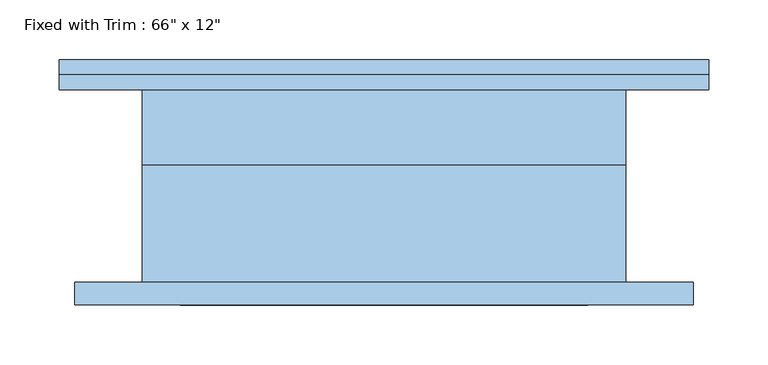
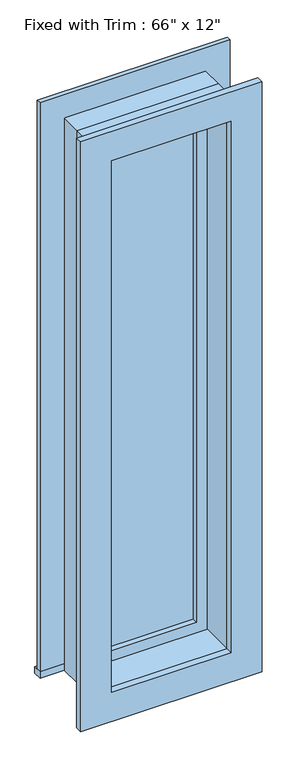
"""IFC4 building model written with IfcOpenShell, lengths in millimetres: window geometry."""

from ifc_helpers import new_model, si_unit, frame, origin, place, context, project, spatial, polyline, outline, extrude, source, transform, mapped, element, save


def window_78a8b392(model_context):
    return source(origin(), model_context, "Body", "SweptSolid", [
        extrude(outline(polyline([(-311.15, 106.3625), (234.95, 106.3625), (234.95, 80.9625), (-311.15, 80.9625), (-311.15, 106.3625)])), frame((0.0, 0.0, 304.8), z_axis=(0.0, 0.0, 1.0), x_axis=(1.0, 0.0, 0.0)), (0.0, 0.0, 1.0), 19.05),
        extrude(outline(polyline([(1962.15, -222.25), (1962.15, 146.05), (323.85, 146.05), (323.85, 234.95), (2051.05, 234.95), (2051.05, -311.15), (323.85, -311.15), (323.85, -222.25), (1962.15, -222.25)])), frame((0.0, 80.9625, 0.0), z_axis=(0.0, 1.0, 0.0), x_axis=(0.0, 0.0, 1.0)), (0.0, 0.0, 1.0), 12.7),
        extrude(outline(polyline([(2038.35, 222.25), (2038.35, -298.45), (247.65, -298.45), (247.65, 222.25), (2038.35, 222.25)]), holes=[polyline([(1949.45, 133.35), (336.55, 133.35), (336.55, -209.55), (1949.45, -209.55), (1949.45, 133.35)])]), frame((0.0, -100.0125, 0.0), z_axis=(0.0, 1.0, 0.0), x_axis=(0.0, 0.0, 1.0)), (0.0, 0.0, 1.0), 19.05),
        extrude(outline(polyline([(101.6, 33.3375), (-177.8, 33.3375), (-177.8, 46.0375), (101.6, 46.0375), (101.6, 33.3375)])), frame((0.0, 0.0, 368.3), z_axis=(0.0, 0.0, 1.0), x_axis=(1.0, 0.0, 0.0)), (0.0, 0.0, 1.0), 1549.4),
        extrude(outline(polyline([(1962.15, -222.25), (323.85, -222.25), (323.85, 146.05), (1962.15, 146.05), (1962.15, -222.25)]), holes=[polyline([(1917.7, -177.8), (1917.7, 101.6), (368.3, 101.6), (368.3, -177.8), (1917.7, -177.8)])]), frame((0.0, 17.4625, 0.0), z_axis=(0.0, 1.0, 0.0), x_axis=(0.0, 0.0, 1.0)), (0.0, 0.0, 1.0), 44.45),
        extrude(outline(polyline([(1981.2, -241.3), (304.8, -241.3), (304.8, 165.1), (1981.2, 165.1), (1981.2, -241.3)]), holes=[polyline([(1949.45, -209.55), (1949.45, 133.35), (336.55, 133.35), (336.55, -209.55), (1949.45, -209.55)])]), frame((0.0, -80.9625, 0.0), z_axis=(0.0, 1.0, 0.0), x_axis=(0.0, 0.0, 1.0)), (0.0, 0.0, 1.0), 98.425),
        extrude(outline(polyline([(1981.2, 165.1), (1981.2, -241.3), (304.8, -241.3), (304.8, 165.1), (1981.2, 165.1)]), holes=[polyline([(1962.15, 146.05), (323.85, 146.05), (323.85, -222.25), (1962.15, -222.25), (1962.15, 146.05)])]), frame((0.0, 17.4625, 0.0), z_axis=(0.0, 1.0, 0.0), x_axis=(0.0, 0.0, 1.0)), (0.0, 0.0, 1.0), 63.5),
    ])


if __name__ == "__main__":
    model = new_model("IFC4")
    model_context = context("Model", 3, world=origin())
    ifc_project = project(units=[si_unit("LENGTHUNIT", "METRE", prefix="MILLI")], contexts=[model_context])
    site = spatial("IfcSite", under=ifc_project)
    building = spatial("IfcBuilding", under=site)
    placement = place(None, origin())
    window_shape = window_78a8b392(model_context)
    element("IfcWindow", 1, ObjectType="Fixed with Trim : 66\" x 12\"", at=placement, inside=building, context=model_context, shape_type="MappedRepresentation", body=[
        mapped(window_shape, transform((0.0, 0.0, 0.0), x_axis=(1.0, 0.0, 0.0), y_axis=(0.0, 1.0, 0.0), z_axis=(0.0, 0.0, 1.0))),
    ])
    save(model, "model.ifc")

# Revit data of these elements
# Type "Fixed with Trim : 66\" x 12\""
#   Type Mark = "54"
#   COBie.Type.CreatedBy = "doug.wood@us.ibm.com"
#   COBie.Type.CreatedOn = "2016-04-14T02:07:26"
#   COBie.Type.Name = "Windows_Fixed with Trim_66\" x 12\"_54"
#   COBie.Type.Category = "23-30 20 17 11 : Fixed Windows"
#   COBie.Type.Description = "Fixed with Trim_66\" x 12\""
#   COBie.Type.Manufacturer = ""
#   COBie.Type.ModelNumber = ""
#   Construction Type Id = "GSP4R"
#   Assembly Code = "B2020100"
#   Analytic Construction = "1/8 in Pilkington single glazing"
#   COBie.Type.ReplacementCost = 0
#   Visual Light Transmittance = 0.9
#   Solar Heat Gain Coefficient = 0.78
#   Heat Transfer Coefficient (U) = 3.6886 W/(m²·K)
#   Height = 5' - 6"
#   Default Sill Height = 1' - 0"
#   Trim Projection - Ext. = 0' - 0 1/2"
#   Trim Projection - Int. = 0' - 0 3/4"
#   Trim Width - Exterior = 0' - 3 1/2"
#   Trim Width - Interior = 0' - 3 1/2"
#   Width = 1' - 4"
#   Window Inset = 0' - 0 3/4"
#   COBie.Type = no
#   Glass Pane Material = Glass
#   Sash Material = Sash - White
#   Trim Exterior Material = Trim - White
#   Trim Interior Material = Trim - White
#   Wall Closure = (empty or 0)
# Element 1 (IfcWindow, "Fixed with Trim : 66\" x 12\"")
#   Materials on its faces: "Sash - White", "Trim - White", "Glass"
# Materials
#   "Glass": class "Glass", colour RGB 0 128 192, transparency 0.75, Description = "Soda Lime Glass", Cost = 0
#   "Sash - White": class "Wood", colour RGB 255 255 255, transparency 0, Cost = 0
#   "Trim - White": class "Wood", colour RGB 255 255 255, transparency 0, Cost = 0
